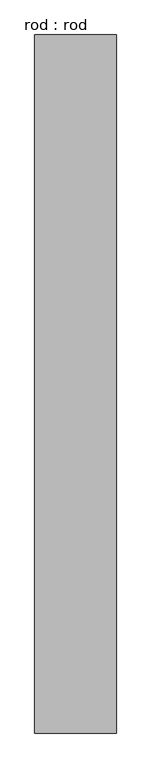
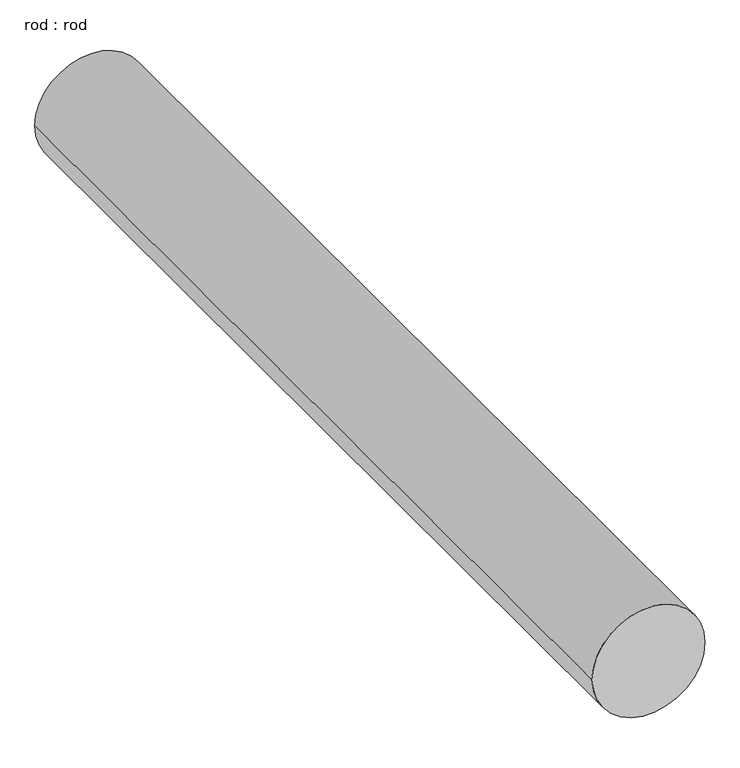
"""IFC4 building model written with IfcOpenShell, lengths in millimetres: proxy geometry, rod : rod."""

import ifcopenshell
import ifcopenshell.guid

model = None  # the IFC model being written
_history = None  # IfcOwnerHistory: only IFC2X3 demands one
_inside = {}  # id of a spatial element -> (the spatial element, [elements in it])
_under = {}  # id of a project, library or spatial element -> (it, [spatial elements below it])
_declared = {}  # id of a project -> (the project, [libraries it declares])
_typed = {}  # id of a type object -> (the type object, [elements of that type])
_made_of = {}  # id of a material, layer set ... -> (it, [elements and type objects made of it])


def new_model(schema):
    """Start an empty IFC model of exactly this schema.

    Asked for "IFC4X3", IfcOpenShell would pick the latest addendum, in which some entities
    have other attributes; the version numbers below select the first issue.
    IFC2X3 requires an IfcOwnerHistory on every rooted entity: one is made here for all.
    """
    global model, _history
    if schema == "IFC4X3":
        model = ifcopenshell.file(schema_version=(4, 3, 0, 0))
    else:
        model = ifcopenshell.file(schema=schema)
    _inside.clear()
    _under.clear()
    _declared.clear()
    _typed.clear()
    _made_of.clear()
    _history = None
    if model.schema == "IFC2X3":
        org = make("IfcOrganization", Name="unknown")
        user = make(
            "IfcPersonAndOrganization",
            ThePerson=make("IfcPerson", FamilyName="unknown"),
            TheOrganization=org,
        )
        app = make(
            "IfcApplication",
            ApplicationDeveloper=org,
            Version="unknown",
            ApplicationFullName="unknown",
            ApplicationIdentifier="unknown",
        )
        _history = make(
            "IfcOwnerHistory",
            OwningUser=user,
            OwningApplication=app,
            ChangeAction="ADDED",
            CreationDate=0,
        )
    return model


def make(cls, **values):
    """One entity of the class cls with the attributes given. An attribute that is None is left unset."""
    return model.create_entity(
        cls, **{name: value for name, value in values.items() if value is not None}
    )


def rooted(cls, **values):
    """An entity with a GlobalId (a new one), such as an element, a storey or a relation."""
    return make(cls, GlobalId=ifcopenshell.guid.new(), OwnerHistory=_history, **values)


def si_unit(unit_type, name, prefix=None):
    """IfcSIUnit, for example si_unit("LENGTHUNIT", "METRE", prefix="MILLI")."""
    return make("IfcSIUnit", UnitType=unit_type, Prefix=prefix, Name=name)


def assignment(units):
    """IfcUnitAssignment: the units of a project."""
    return None if units is None else make("IfcUnitAssignment", Units=units)


def point(xyz):
    """IfcCartesianPoint."""
    return None if xyz is None else make("IfcCartesianPoint", Coordinates=xyz)


def direction(xyz):
    """IfcDirection."""
    return None if xyz is None else make("IfcDirection", DirectionRatios=xyz)


def frame(location, z_axis=None, x_axis=None):
    """IfcAxis2Placement3D, a coordinate frame: its origin and axes. An axis left out is left unset."""
    return make(
        "IfcAxis2Placement3D",
        Location=point(location),
        Axis=direction(z_axis),
        RefDirection=direction(x_axis),
    )


def frame_2d(location, x_axis=None):
    """IfcAxis2Placement2D, a coordinate frame in the plane: its origin and x axis."""
    return make(
        "IfcAxis2Placement2D", Location=point(location), RefDirection=direction(x_axis)
    )


def origin():
    """The frame at (0, 0, 0) with its axes left unset."""
    return frame((0.0, 0.0, 0.0))


def place(relative_to, where):
    """IfcLocalPlacement: puts the frame where relative to a parent placement (None: the world)."""
    return make(
        "IfcLocalPlacement", PlacementRelTo=relative_to, RelativePlacement=where
    )


def context(
    kind, dimensions, precision=None, world=None, true_north=None, identifier=None
):
    """IfcGeometricRepresentationContext, for example the 3D "Model" context."""
    return make(
        "IfcGeometricRepresentationContext",
        ContextIdentifier=identifier,
        ContextType=kind,
        CoordinateSpaceDimension=dimensions,
        Precision=precision,
        WorldCoordinateSystem=world,
        TrueNorth=true_north,
    )


def project(units=None, contexts=None):
    """IfcProject with its units and contexts."""
    return rooted(
        "IfcProject",
        Name="project",
        RepresentationContexts=contexts,
        UnitsInContext=assignment(units),
    )


def spatial(cls, under=None, at=None, **own):
    """A site, building, storey or space (cls), placed at a placement, below another one or the project."""
    s = rooted(cls, ObjectPlacement=at, **own)
    if under is not None:
        _under.setdefault(under.id(), (under, []))[1].append(s)
    return s


def circle_curve(where, radius):
    """IfcCircle in the frame where."""
    return make("IfcCircle", Position=where, Radius=radius)


def trimmed(basis, trim1, trim2, sense, master):
    """IfcTrimmedCurve: the piece of a basis curve between two trims."""
    return make(
        "IfcTrimmedCurve",
        BasisCurve=basis,
        Trim1=trim1,
        Trim2=trim2,
        SenseAgreement=sense,
        MasterRepresentation=master,
    )


def segment(curve, same_sense, transition):
    """IfcCompositeCurveSegment."""
    return make(
        "IfcCompositeCurveSegment",
        Transition=transition,
        SameSense=same_sense,
        ParentCurve=curve,
    )


def composite_curve(segments, self_intersect=None):
    """IfcCompositeCurve: segments joined end to end."""
    return make("IfcCompositeCurve", Segments=segments, SelfIntersect=self_intersect)


def outline(outer, holes=None, kind="AREA"):
    """IfcArbitraryClosedProfileDef: a profile drawn as a closed curve; with holes, ...WithVoids."""
    if holes is None:
        return make("IfcArbitraryClosedProfileDef", ProfileType=kind, OuterCurve=outer)
    return make(
        "IfcArbitraryProfileDefWithVoids",
        ProfileType=kind,
        OuterCurve=outer,
        InnerCurves=holes,
    )


def extrude(swept, where, along, depth):
    """IfcExtrudedAreaSolid: the profile swept, set in the frame where, extruded along a direction by depth."""
    return make(
        "IfcExtrudedAreaSolid",
        SweptArea=swept,
        Position=where,
        ExtrudedDirection=direction(along),
        Depth=depth,
    )


def shape(context_of_items, identifier, shape_type, items):
    """IfcShapeRepresentation: the items that make up one representation, for example the "Body"."""
    return make(
        "IfcShapeRepresentation",
        ContextOfItems=context_of_items,
        RepresentationIdentifier=identifier,
        RepresentationType=shape_type,
        Items=items,
    )


def source(mapping_origin, context_of_items, identifier, shape_type, items):
    """IfcRepresentationMap: a shape defined once, which mapped items show again and again."""
    return make(
        "IfcRepresentationMap",
        MappingOrigin=mapping_origin,
        MappedRepresentation=shape(context_of_items, identifier, shape_type, items),
    )


def transform(
    local_origin,
    x_axis=None,
    y_axis=None,
    z_axis=None,
    scale=None,
    scale2=None,
    scale3=None,
    uniform=True,
):
    """IfcCartesianTransformationOperator3D, or its non-uniform kind. x_axis, y_axis, z_axis: its Axis1, 2, 3."""
    if uniform:
        return make(
            "IfcCartesianTransformationOperator3D",
            Axis1=direction(x_axis),
            Axis2=direction(y_axis),
            LocalOrigin=point(local_origin),
            Scale=scale,
            Axis3=direction(z_axis),
        )
    return make(
        "IfcCartesianTransformationOperator3DnonUniform",
        Axis1=direction(x_axis),
        Axis2=direction(y_axis),
        LocalOrigin=point(local_origin),
        Scale=scale,
        Axis3=direction(z_axis),
        Scale2=scale2,
        Scale3=scale3,
    )


def mapped(mapping_source, mapping_target):
    """IfcMappedItem: shows the shape of a source again, moved by a transform."""
    return make(
        "IfcMappedItem", MappingSource=mapping_source, MappingTarget=mapping_target
    )


def made_of(thing, what):
    """Note that an element or type object is made of a material, layer set ...; save() writes the relation."""
    if what is not None:
        _made_of.setdefault(what.id(), (what, []))[1].append(thing)
    return thing


def element(
    cls,
    number,
    at=None,
    inside=None,
    cuts=None,
    type_object=None,
    material=None,
    context=None,
    identifier="Body",
    shape_type=None,
    held_by="IfcProductDefinitionShape",
    body=None,
    shapes=None,
    **own,
):
    """One element of the class cls, such as IfcWall. Its Tag is "e" and its number.

    at: its placement. inside: the storey or other place that contains it. cuts: it is an
    opening in that element (IfcRelVoidsElement). A single representation is given by context,
    identifier, shape_type and body (its items); several are given by shapes. held_by: the class
    of the entity that holds the representations. save() writes the other relations.
    """
    e = rooted(cls, Tag="e%d" % number, ObjectPlacement=at, **own)
    if body is not None:
        shapes = [shape(context, identifier, shape_type, body)]
    if shapes is not None:
        e.Representation = make(held_by, Representations=shapes)
    if inside is not None:
        _inside.setdefault(inside.id(), (inside, []))[1].append(e)
    if cuts is not None:
        rooted(
            "IfcRelVoidsElement", RelatingBuildingElement=cuts, RelatedOpeningElement=e
        )
    if type_object is not None:
        _typed.setdefault(type_object.id(), (type_object, []))[1].append(e)
    return made_of(e, material)


def aggregate(whole, parts):
    """IfcRelAggregates: a whole, such as a stair, and the parts it consists of."""
    return rooted("IfcRelAggregates", RelatingObject=whole, RelatedObjects=parts)


def save(model, path):
    """Write the relations noted so far, then the file.

    IfcRelAggregates (storeys below a building ...), IfcRelContainedInSpatialStructure (elements
    in a storey), IfcRelDefinesByType, IfcRelAssociatesMaterial and IfcRelDeclares: one each for
    every whole, place, type object, material and project.
    """
    for whole, parts in _under.values():
        aggregate(whole, parts)
    for where, things in _inside.values():
        rooted(
            "IfcRelContainedInSpatialStructure",
            RelatedElements=things,
            RelatingStructure=where,
        )
    for kind, things in _typed.values():
        rooted("IfcRelDefinesByType", RelatedObjects=things, RelatingType=kind)
    for what, things in _made_of.values():
        rooted("IfcRelAssociatesMaterial", RelatedObjects=things, RelatingMaterial=what)
    for by, libraries in _declared.values():
        rooted("IfcRelDeclares", RelatingContext=by, RelatedDefinitions=libraries)
    model.write(path)


def rod_rod_a14e13bd(model_context):
    return source(origin(), model_context, "Body", "SweptSolid", [
        extrude(outline(composite_curve([segment(trimmed(circle_curve(frame_2d((0.0108462, 0.0)), 200.0), [point((0.0108462, 200.0))], [point((0.0108462, -200.0))], False, "CARTESIAN"), True, "CONTINUOUS"), segment(trimmed(circle_curve(frame_2d((0.0108462, 0.0)), 200.0), [point((0.0108462, -200.0))], [point((0.0108462, 200.0))], False, "CARTESIAN"), True, "CONTINUOUS")], self_intersect=False)), frame((0.0, 2382.7286153, 0.0), z_axis=(0.0, 1.0, 0.0), x_axis=(0.0, 0.0, 1.0)), (0.0, 0.0, 1.0), 3420.0),
    ])


if __name__ == "__main__":
    model = new_model("IFC4")
    model_context = context("Model", 3, world=origin())
    ifc_project = project(units=[si_unit("LENGTHUNIT", "METRE", prefix="MILLI")], contexts=[model_context])
    site = spatial("IfcSite", under=ifc_project)
    building = spatial("IfcBuilding", under=site)
    placement = place(None, origin())
    rod_rod_shape = rod_rod_a14e13bd(model_context)
    element("IfcBuildingElementProxy", 1, Name="rod : rod", ObjectType="rod : rod", at=placement, inside=building, context=model_context, shape_type="MappedRepresentation", body=[
        mapped(rod_rod_shape, transform((0.0, 0.0, 0.0), x_axis=(1.0, 0.0, 0.0), y_axis=(0.0, 1.0, 0.0), z_axis=(0.0, 0.0, 1.0))),
    ])
    save(model, "model.ifc")

# Revit data of these elements
# Type "rod : rod"
#   Default Elevation = 0
